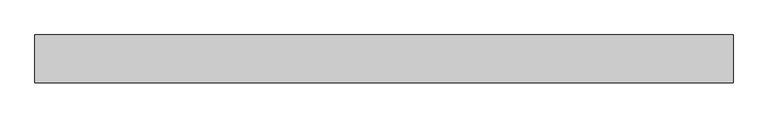
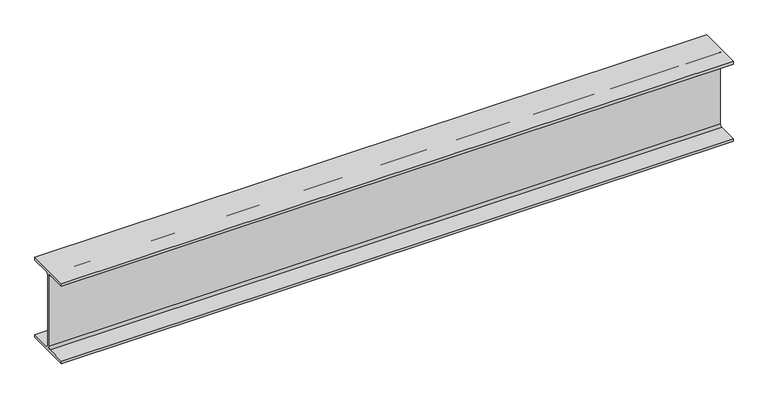
"""IFC4 building model written with IfcOpenShell, lengths in millimetres: beam geometry, Old_Steel Beam_H-KSD3502 : H_SB_ASB_H-200×200x8x12."""

import ifcopenshell
import ifcopenshell.guid

model = None  # the IFC model being written
_history = None  # IfcOwnerHistory: only IFC2X3 demands one
_inside = {}  # id of a spatial element -> (the spatial element, [elements in it])
_under = {}  # id of a project, library or spatial element -> (it, [spatial elements below it])
_declared = {}  # id of a project -> (the project, [libraries it declares])
_typed = {}  # id of a type object -> (the type object, [elements of that type])
_made_of = {}  # id of a material, layer set ... -> (it, [elements and type objects made of it])


def new_model(schema):
    """Start an empty IFC model of exactly this schema.

    Asked for "IFC4X3", IfcOpenShell would pick the latest addendum, in which some entities
    have other attributes; the version numbers below select the first issue.
    IFC2X3 requires an IfcOwnerHistory on every rooted entity: one is made here for all.
    """
    global model, _history
    if schema == "IFC4X3":
        model = ifcopenshell.file(schema_version=(4, 3, 0, 0))
    else:
        model = ifcopenshell.file(schema=schema)
    _inside.clear()
    _under.clear()
    _declared.clear()
    _typed.clear()
    _made_of.clear()
    _history = None
    if model.schema == "IFC2X3":
        org = make("IfcOrganization", Name="unknown")
        user = make(
            "IfcPersonAndOrganization",
            ThePerson=make("IfcPerson", FamilyName="unknown"),
            TheOrganization=org,
        )
        app = make(
            "IfcApplication",
            ApplicationDeveloper=org,
            Version="unknown",
            ApplicationFullName="unknown",
            ApplicationIdentifier="unknown",
        )
        _history = make(
            "IfcOwnerHistory",
            OwningUser=user,
            OwningApplication=app,
            ChangeAction="ADDED",
            CreationDate=0,
        )
    return model


def make(cls, **values):
    """One entity of the class cls with the attributes given. An attribute that is None is left unset."""
    return model.create_entity(
        cls, **{name: value for name, value in values.items() if value is not None}
    )


def rooted(cls, **values):
    """An entity with a GlobalId (a new one), such as an element, a storey or a relation."""
    return make(cls, GlobalId=ifcopenshell.guid.new(), OwnerHistory=_history, **values)


def si_unit(unit_type, name, prefix=None):
    """IfcSIUnit, for example si_unit("LENGTHUNIT", "METRE", prefix="MILLI")."""
    return make("IfcSIUnit", UnitType=unit_type, Prefix=prefix, Name=name)


def assignment(units):
    """IfcUnitAssignment: the units of a project."""
    return None if units is None else make("IfcUnitAssignment", Units=units)


def point(xyz):
    """IfcCartesianPoint."""
    return None if xyz is None else make("IfcCartesianPoint", Coordinates=xyz)


def direction(xyz):
    """IfcDirection."""
    return None if xyz is None else make("IfcDirection", DirectionRatios=xyz)


def frame(location, z_axis=None, x_axis=None):
    """IfcAxis2Placement3D, a coordinate frame: its origin and axes. An axis left out is left unset."""
    return make(
        "IfcAxis2Placement3D",
        Location=point(location),
        Axis=direction(z_axis),
        RefDirection=direction(x_axis),
    )


def frame_2d(location, x_axis=None):
    """IfcAxis2Placement2D, a coordinate frame in the plane: its origin and x axis."""
    return make(
        "IfcAxis2Placement2D", Location=point(location), RefDirection=direction(x_axis)
    )


def origin():
    """The frame at (0, 0, 0) with its axes left unset."""
    return frame((0.0, 0.0, 0.0))


def place(relative_to, where):
    """IfcLocalPlacement: puts the frame where relative to a parent placement (None: the world)."""
    return make(
        "IfcLocalPlacement", PlacementRelTo=relative_to, RelativePlacement=where
    )


def context(
    kind, dimensions, precision=None, world=None, true_north=None, identifier=None
):
    """IfcGeometricRepresentationContext, for example the 3D "Model" context."""
    return make(
        "IfcGeometricRepresentationContext",
        ContextIdentifier=identifier,
        ContextType=kind,
        CoordinateSpaceDimension=dimensions,
        Precision=precision,
        WorldCoordinateSystem=world,
        TrueNorth=true_north,
    )


def project(units=None, contexts=None):
    """IfcProject with its units and contexts."""
    return rooted(
        "IfcProject",
        Name="project",
        RepresentationContexts=contexts,
        UnitsInContext=assignment(units),
    )


def spatial(cls, under=None, at=None, **own):
    """A site, building, storey or space (cls), placed at a placement, below another one or the project."""
    s = rooted(cls, ObjectPlacement=at, **own)
    if under is not None:
        _under.setdefault(under.id(), (under, []))[1].append(s)
    return s


def polyline(points):
    """IfcPolyline through the points."""
    return make("IfcPolyline", Points=[point(p) for p in points])


def circle_curve(where, radius):
    """IfcCircle in the frame where."""
    return make("IfcCircle", Position=where, Radius=radius)


def trimmed(basis, trim1, trim2, sense, master):
    """IfcTrimmedCurve: the piece of a basis curve between two trims."""
    return make(
        "IfcTrimmedCurve",
        BasisCurve=basis,
        Trim1=trim1,
        Trim2=trim2,
        SenseAgreement=sense,
        MasterRepresentation=master,
    )


def segment(curve, same_sense, transition):
    """IfcCompositeCurveSegment."""
    return make(
        "IfcCompositeCurveSegment",
        Transition=transition,
        SameSense=same_sense,
        ParentCurve=curve,
    )


def composite_curve(segments, self_intersect=None):
    """IfcCompositeCurve: segments joined end to end."""
    return make("IfcCompositeCurve", Segments=segments, SelfIntersect=self_intersect)


def outline(outer, holes=None, kind="AREA"):
    """IfcArbitraryClosedProfileDef: a profile drawn as a closed curve; with holes, ...WithVoids."""
    if holes is None:
        return make("IfcArbitraryClosedProfileDef", ProfileType=kind, OuterCurve=outer)
    return make(
        "IfcArbitraryProfileDefWithVoids",
        ProfileType=kind,
        OuterCurve=outer,
        InnerCurves=holes,
    )


def extrude(swept, where, along, depth):
    """IfcExtrudedAreaSolid: the profile swept, set in the frame where, extruded along a direction by depth."""
    return make(
        "IfcExtrudedAreaSolid",
        SweptArea=swept,
        Position=where,
        ExtrudedDirection=direction(along),
        Depth=depth,
    )


def shape(context_of_items, identifier, shape_type, items):
    """IfcShapeRepresentation: the items that make up one representation, for example the "Body"."""
    return make(
        "IfcShapeRepresentation",
        ContextOfItems=context_of_items,
        RepresentationIdentifier=identifier,
        RepresentationType=shape_type,
        Items=items,
    )


def source(mapping_origin, context_of_items, identifier, shape_type, items):
    """IfcRepresentationMap: a shape defined once, which mapped items show again and again."""
    return make(
        "IfcRepresentationMap",
        MappingOrigin=mapping_origin,
        MappedRepresentation=shape(context_of_items, identifier, shape_type, items),
    )


def transform(
    local_origin,
    x_axis=None,
    y_axis=None,
    z_axis=None,
    scale=None,
    scale2=None,
    scale3=None,
    uniform=True,
):
    """IfcCartesianTransformationOperator3D, or its non-uniform kind. x_axis, y_axis, z_axis: its Axis1, 2, 3."""
    if uniform:
        return make(
            "IfcCartesianTransformationOperator3D",
            Axis1=direction(x_axis),
            Axis2=direction(y_axis),
            LocalOrigin=point(local_origin),
            Scale=scale,
            Axis3=direction(z_axis),
        )
    return make(
        "IfcCartesianTransformationOperator3DnonUniform",
        Axis1=direction(x_axis),
        Axis2=direction(y_axis),
        LocalOrigin=point(local_origin),
        Scale=scale,
        Axis3=direction(z_axis),
        Scale2=scale2,
        Scale3=scale3,
    )


def mapped(mapping_source, mapping_target):
    """IfcMappedItem: shows the shape of a source again, moved by a transform."""
    return make(
        "IfcMappedItem", MappingSource=mapping_source, MappingTarget=mapping_target
    )


def made_of(thing, what):
    """Note that an element or type object is made of a material, layer set ...; save() writes the relation."""
    if what is not None:
        _made_of.setdefault(what.id(), (what, []))[1].append(thing)
    return thing


def element(
    cls,
    number,
    at=None,
    inside=None,
    cuts=None,
    type_object=None,
    material=None,
    context=None,
    identifier="Body",
    shape_type=None,
    held_by="IfcProductDefinitionShape",
    body=None,
    shapes=None,
    **own,
):
    """One element of the class cls, such as IfcWall. Its Tag is "e" and its number.

    at: its placement. inside: the storey or other place that contains it. cuts: it is an
    opening in that element (IfcRelVoidsElement). A single representation is given by context,
    identifier, shape_type and body (its items); several are given by shapes. held_by: the class
    of the entity that holds the representations. save() writes the other relations.
    """
    e = rooted(cls, Tag="e%d" % number, ObjectPlacement=at, **own)
    if body is not None:
        shapes = [shape(context, identifier, shape_type, body)]
    if shapes is not None:
        e.Representation = make(held_by, Representations=shapes)
    if inside is not None:
        _inside.setdefault(inside.id(), (inside, []))[1].append(e)
    if cuts is not None:
        rooted(
            "IfcRelVoidsElement", RelatingBuildingElement=cuts, RelatedOpeningElement=e
        )
    if type_object is not None:
        _typed.setdefault(type_object.id(), (type_object, []))[1].append(e)
    return made_of(e, material)


def aggregate(whole, parts):
    """IfcRelAggregates: a whole, such as a stair, and the parts it consists of."""
    return rooted("IfcRelAggregates", RelatingObject=whole, RelatedObjects=parts)


def save(model, path):
    """Write the relations noted so far, then the file.

    IfcRelAggregates (storeys below a building ...), IfcRelContainedInSpatialStructure (elements
    in a storey), IfcRelDefinesByType, IfcRelAssociatesMaterial and IfcRelDeclares: one each for
    every whole, place, type object, material and project.
    """
    for whole, parts in _under.values():
        aggregate(whole, parts)
    for where, things in _inside.values():
        rooted(
            "IfcRelContainedInSpatialStructure",
            RelatedElements=things,
            RelatingStructure=where,
        )
    for kind, things in _typed.values():
        rooted("IfcRelDefinesByType", RelatedObjects=things, RelatingType=kind)
    for what, things in _made_of.values():
        rooted("IfcRelAssociatesMaterial", RelatedObjects=things, RelatingMaterial=what)
    for by, libraries in _declared.values():
        rooted("IfcRelDeclares", RelatingContext=by, RelatedDefinitions=libraries)
    model.write(path)


def beam_92807fc5(model_context):
    return source(origin(), model_context, "Body", "SweptSolid", [
        extrude(outline(composite_curve([segment(polyline([(82.5, -141.5), (82.5, -151.7), (-82.5, -151.7), (-82.5, -141.5), (-11.9, -141.5)]), True, "CONTINUOUS"), segment(trimmed(circle_curve(frame_2d((-11.9, -132.6)), 8.9), [point((-11.9, -141.5))], [point((-3.0, -132.6))], True, "CARTESIAN"), True, "CONTINUOUS"), segment(polyline([(-3.0, -132.6), (-3.0, 132.6)]), True, "CONTINUOUS"), segment(trimmed(circle_curve(frame_2d((-11.9, 132.6)), 8.9), [point((-3.0, 132.6))], [point((-11.9, 141.5))], True, "CARTESIAN"), True, "CONTINUOUS"), segment(polyline([(-11.9, 141.5), (-82.5, 141.5), (-82.5, 151.7), (82.5, 151.7), (82.5, 141.5), (11.9, 141.5)]), True, "CONTINUOUS"), segment(trimmed(circle_curve(frame_2d((11.9, 132.6)), 8.9), [point((11.9, 141.5))], [point((3.0, 132.6))], True, "CARTESIAN"), True, "CONTINUOUS"), segment(polyline([(3.0, 132.6), (3.0, -132.6)]), True, "CONTINUOUS"), segment(trimmed(circle_curve(frame_2d((11.9, -132.6)), 8.9), [point((3.0, -132.6))], [point((11.9, -141.5))], True, "CARTESIAN"), True, "CONTINUOUS"), segment(polyline([(11.9, -141.5), (82.5, -141.5)]), True, "CONTINUOUS")], self_intersect=False)), frame((-1199.8807155, 0.0, 0.0), z_axis=(1.0, 0.0, 0.0), x_axis=(0.0, 1.0, 0.0)), (0.0, 0.0, 1.0), 2406.4861403),
    ])


if __name__ == "__main__":
    model = new_model("IFC4")
    model_context = context("Model", 3, world=origin())
    ifc_project = project(units=[si_unit("LENGTHUNIT", "METRE", prefix="MILLI")], contexts=[model_context])
    site = spatial("IfcSite", under=ifc_project)
    building = spatial("IfcBuilding", under=site)
    placement = place(None, origin())
    beam_shape = beam_92807fc5(model_context)
    element("IfcBeam", 1, ObjectType="Old_Steel Beam_H-KSD3502 : H_SB_ASB_H-200×200x8x12", at=placement, inside=building, context=model_context, shape_type="MappedRepresentation", body=[
        mapped(beam_shape, transform((0.0, 0.0, 0.0), x_axis=(1.0, 0.0, 0.0), y_axis=(0.0, 1.0, 0.0), z_axis=(0.0, 0.0, 1.0))),
    ])
    save(model, "model.ifc")

# Revit data of these elements
# Type "Old_Steel Beam_H-KSD3502 : H_SB_ASB_H-200×200x8x12"
#   Width = 20.0 cm
#   Web Thickness = 0.8 cm
#   Web Fillet = 1.3 cm
#   Warping Constant = 141376.0 cm⁶
#   Torsional Moment of Inertia = 26.2485 cm⁴
#   Torsional Modulus = 1.0 cm³
#   Section Area = 63.53 cm²
#   Plastic Modulus weak axis = 244.0 cm³
#   Plastic Modulus strong axis = 525.0 cm³
#   Perimeter = 1.16 m²/m
#   Nominal Weight = 49.90 kgf/m
#   Moment of Inertia weak axis = 1600.00 cm⁴
#   Moment of Inertia strong axis = 4720.00 cm⁴
#   Height = 20.0 cm
#   Flange Thickness = 1.2 cm
#   Elastic Modulus weak axis = 160.0 cm³
#   Elastic Modulus strong axis = 472.0 cm³
#   Centroid Vertical = 10.0 cm
#   Centroid Horizontal = 10.0 cm
#   Length [instance default] = 1.5240 m
#   Structural Material [instance default] = Steel, 45-345
#   Assembly Code = ""
# Element 1 (IfcBeam, "Old_Steel Beam_H-KSD3502 : H_SB_ASB_H-200×200x8x12")
#   Structural Material = none
# Materials
#   "Steel, 45-345": class "Metal", colour RGB 189 187 185, transparency 0, Description = "Steel 345 MPa", Cost = 0
